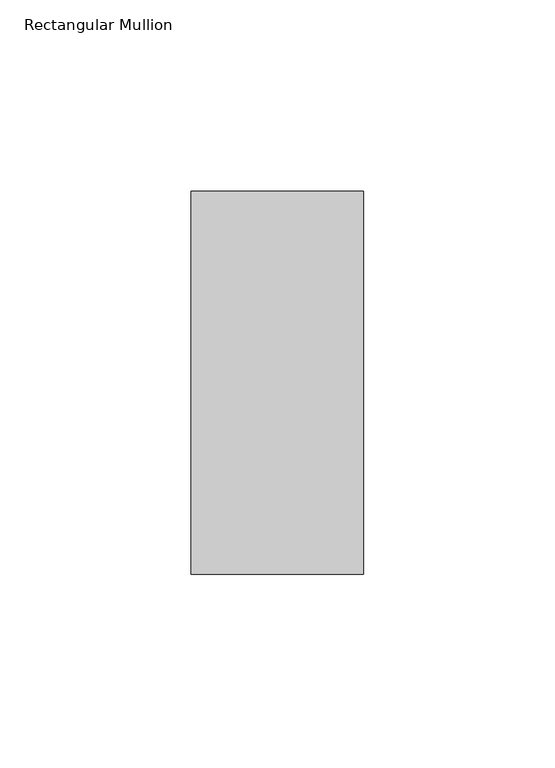
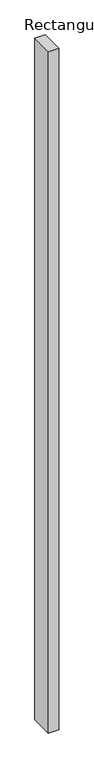
"""IFC4 building model written with IfcOpenShell, lengths in millimetres: member geometry, Rectangular Mullion : 알루미늄_Rectangular Cap_100 x 45."""

from ifc_helpers import new_model, si_unit, frame, origin, place, context, project, spatial, polyline, outline, extrude, source, transform, mapped, element, save


def rectangular_mullion_35e44d10(model_context):
    return source(origin(), model_context, "Body", "SweptSolid", [
        extrude(outline(polyline([(0.0, 50.0), (0.0, -50.0), (-45.0, -50.0), (-45.0, 50.0), (0.0, 50.0)])), frame((0.0, 0.0, -3100.0), z_axis=(0.0, 0.0, 1.0), x_axis=(1.0, 0.0, 0.0)), (0.0, 0.0, 1.0), 3100.0),
    ])


if __name__ == "__main__":
    model = new_model("IFC4")
    model_context = context("Model", 3, world=origin())
    ifc_project = project(units=[si_unit("LENGTHUNIT", "METRE", prefix="MILLI")], contexts=[model_context])
    site = spatial("IfcSite", under=ifc_project)
    building = spatial("IfcBuilding", under=site)
    placement = place(None, origin())
    rectangular_mullion_shape = rectangular_mullion_35e44d10(model_context)
    element("IfcMember", 1, ObjectType="Rectangular Mullion : 알루미늄_Rectangular Cap_100 x 45", at=placement, inside=building, context=model_context, shape_type="MappedRepresentation", body=[
        mapped(rectangular_mullion_shape, transform((0.0, 0.0, 0.0), x_axis=(1.0, 0.0, 0.0), y_axis=(0.0, 1.0, 0.0), z_axis=(0.0, 0.0, 1.0))),
    ])
    save(model, "model.ifc")

# Revit data of these elements
# Type "Rectangular Mullion : 알루미늄_Rectangular Cap_100 x 45"
#   built-in parameter 1007304 = 0.328084 (stored number, unit not read)
#   built-in parameter 1007301 = 0.0738189 (stored number, unit not read)
#   built-in parameter 1007300 = 0.0738189 (stored number, unit not read)
# Element 1 (IfcMember, "Rectangular Mullion : 알루미늄_Rectangular Cap_100 x 45")
#   Materials on its faces: "00_Metal_Stainless Steel"
# Materials
#   "00_Metal_Stainless Steel": class "Metal", colour RGB 148 148 148, transparency 0, Description = "Steel", Cost = 0
